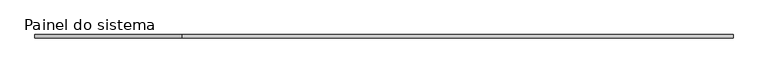
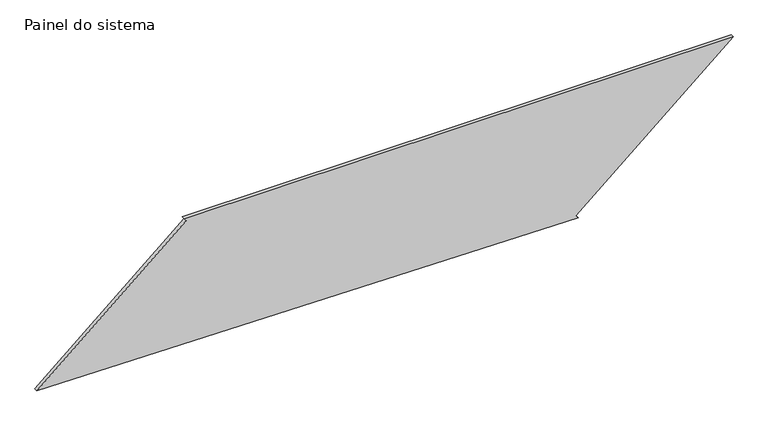
"""IFC4 building model written with IfcOpenShell, lengths in millimetres: plate geometry, Painel do sistema : Envidraçado."""

import ifcopenshell
import ifcopenshell.guid

model = None  # the IFC model being written
_history = None  # IfcOwnerHistory: only IFC2X3 demands one
_inside = {}  # id of a spatial element -> (the spatial element, [elements in it])
_under = {}  # id of a project, library or spatial element -> (it, [spatial elements below it])
_declared = {}  # id of a project -> (the project, [libraries it declares])
_typed = {}  # id of a type object -> (the type object, [elements of that type])
_made_of = {}  # id of a material, layer set ... -> (it, [elements and type objects made of it])


def new_model(schema):
    """Start an empty IFC model of exactly this schema.

    Asked for "IFC4X3", IfcOpenShell would pick the latest addendum, in which some entities
    have other attributes; the version numbers below select the first issue.
    IFC2X3 requires an IfcOwnerHistory on every rooted entity: one is made here for all.
    """
    global model, _history
    if schema == "IFC4X3":
        model = ifcopenshell.file(schema_version=(4, 3, 0, 0))
    else:
        model = ifcopenshell.file(schema=schema)
    _inside.clear()
    _under.clear()
    _declared.clear()
    _typed.clear()
    _made_of.clear()
    _history = None
    if model.schema == "IFC2X3":
        org = make("IfcOrganization", Name="unknown")
        user = make(
            "IfcPersonAndOrganization",
            ThePerson=make("IfcPerson", FamilyName="unknown"),
            TheOrganization=org,
        )
        app = make(
            "IfcApplication",
            ApplicationDeveloper=org,
            Version="unknown",
            ApplicationFullName="unknown",
            ApplicationIdentifier="unknown",
        )
        _history = make(
            "IfcOwnerHistory",
            OwningUser=user,
            OwningApplication=app,
            ChangeAction="ADDED",
            CreationDate=0,
        )
    return model


def make(cls, **values):
    """One entity of the class cls with the attributes given. An attribute that is None is left unset."""
    return model.create_entity(
        cls, **{name: value for name, value in values.items() if value is not None}
    )


def rooted(cls, **values):
    """An entity with a GlobalId (a new one), such as an element, a storey or a relation."""
    return make(cls, GlobalId=ifcopenshell.guid.new(), OwnerHistory=_history, **values)


def si_unit(unit_type, name, prefix=None):
    """IfcSIUnit, for example si_unit("LENGTHUNIT", "METRE", prefix="MILLI")."""
    return make("IfcSIUnit", UnitType=unit_type, Prefix=prefix, Name=name)


def assignment(units):
    """IfcUnitAssignment: the units of a project."""
    return None if units is None else make("IfcUnitAssignment", Units=units)


def point(xyz):
    """IfcCartesianPoint."""
    return None if xyz is None else make("IfcCartesianPoint", Coordinates=xyz)


def direction(xyz):
    """IfcDirection."""
    return None if xyz is None else make("IfcDirection", DirectionRatios=xyz)


def frame(location, z_axis=None, x_axis=None):
    """IfcAxis2Placement3D, a coordinate frame: its origin and axes. An axis left out is left unset."""
    return make(
        "IfcAxis2Placement3D",
        Location=point(location),
        Axis=direction(z_axis),
        RefDirection=direction(x_axis),
    )


def origin():
    """The frame at (0, 0, 0) with its axes left unset."""
    return frame((0.0, 0.0, 0.0))


def place(relative_to, where):
    """IfcLocalPlacement: puts the frame where relative to a parent placement (None: the world)."""
    return make(
        "IfcLocalPlacement", PlacementRelTo=relative_to, RelativePlacement=where
    )


def context(
    kind, dimensions, precision=None, world=None, true_north=None, identifier=None
):
    """IfcGeometricRepresentationContext, for example the 3D "Model" context."""
    return make(
        "IfcGeometricRepresentationContext",
        ContextIdentifier=identifier,
        ContextType=kind,
        CoordinateSpaceDimension=dimensions,
        Precision=precision,
        WorldCoordinateSystem=world,
        TrueNorth=true_north,
    )


def project(units=None, contexts=None):
    """IfcProject with its units and contexts."""
    return rooted(
        "IfcProject",
        Name="project",
        RepresentationContexts=contexts,
        UnitsInContext=assignment(units),
    )


def spatial(cls, under=None, at=None, **own):
    """A site, building, storey or space (cls), placed at a placement, below another one or the project."""
    s = rooted(cls, ObjectPlacement=at, **own)
    if under is not None:
        _under.setdefault(under.id(), (under, []))[1].append(s)
    return s


def polyline(points):
    """IfcPolyline through the points."""
    return make("IfcPolyline", Points=[point(p) for p in points])


def outline(outer, holes=None, kind="AREA"):
    """IfcArbitraryClosedProfileDef: a profile drawn as a closed curve; with holes, ...WithVoids."""
    if holes is None:
        return make("IfcArbitraryClosedProfileDef", ProfileType=kind, OuterCurve=outer)
    return make(
        "IfcArbitraryProfileDefWithVoids",
        ProfileType=kind,
        OuterCurve=outer,
        InnerCurves=holes,
    )


def extrude(swept, where, along, depth):
    """IfcExtrudedAreaSolid: the profile swept, set in the frame where, extruded along a direction by depth."""
    return make(
        "IfcExtrudedAreaSolid",
        SweptArea=swept,
        Position=where,
        ExtrudedDirection=direction(along),
        Depth=depth,
    )


def shape(context_of_items, identifier, shape_type, items):
    """IfcShapeRepresentation: the items that make up one representation, for example the "Body"."""
    return make(
        "IfcShapeRepresentation",
        ContextOfItems=context_of_items,
        RepresentationIdentifier=identifier,
        RepresentationType=shape_type,
        Items=items,
    )


def source(mapping_origin, context_of_items, identifier, shape_type, items):
    """IfcRepresentationMap: a shape defined once, which mapped items show again and again."""
    return make(
        "IfcRepresentationMap",
        MappingOrigin=mapping_origin,
        MappedRepresentation=shape(context_of_items, identifier, shape_type, items),
    )


def transform(
    local_origin,
    x_axis=None,
    y_axis=None,
    z_axis=None,
    scale=None,
    scale2=None,
    scale3=None,
    uniform=True,
):
    """IfcCartesianTransformationOperator3D, or its non-uniform kind. x_axis, y_axis, z_axis: its Axis1, 2, 3."""
    if uniform:
        return make(
            "IfcCartesianTransformationOperator3D",
            Axis1=direction(x_axis),
            Axis2=direction(y_axis),
            LocalOrigin=point(local_origin),
            Scale=scale,
            Axis3=direction(z_axis),
        )
    return make(
        "IfcCartesianTransformationOperator3DnonUniform",
        Axis1=direction(x_axis),
        Axis2=direction(y_axis),
        LocalOrigin=point(local_origin),
        Scale=scale,
        Axis3=direction(z_axis),
        Scale2=scale2,
        Scale3=scale3,
    )


def mapped(mapping_source, mapping_target):
    """IfcMappedItem: shows the shape of a source again, moved by a transform."""
    return make(
        "IfcMappedItem", MappingSource=mapping_source, MappingTarget=mapping_target
    )


def made_of(thing, what):
    """Note that an element or type object is made of a material, layer set ...; save() writes the relation."""
    if what is not None:
        _made_of.setdefault(what.id(), (what, []))[1].append(thing)
    return thing


def element(
    cls,
    number,
    at=None,
    inside=None,
    cuts=None,
    type_object=None,
    material=None,
    context=None,
    identifier="Body",
    shape_type=None,
    held_by="IfcProductDefinitionShape",
    body=None,
    shapes=None,
    **own,
):
    """One element of the class cls, such as IfcWall. Its Tag is "e" and its number.

    at: its placement. inside: the storey or other place that contains it. cuts: it is an
    opening in that element (IfcRelVoidsElement). A single representation is given by context,
    identifier, shape_type and body (its items); several are given by shapes. held_by: the class
    of the entity that holds the representations. save() writes the other relations.
    """
    e = rooted(cls, Tag="e%d" % number, ObjectPlacement=at, **own)
    if body is not None:
        shapes = [shape(context, identifier, shape_type, body)]
    if shapes is not None:
        e.Representation = make(held_by, Representations=shapes)
    if inside is not None:
        _inside.setdefault(inside.id(), (inside, []))[1].append(e)
    if cuts is not None:
        rooted(
            "IfcRelVoidsElement", RelatingBuildingElement=cuts, RelatedOpeningElement=e
        )
    if type_object is not None:
        _typed.setdefault(type_object.id(), (type_object, []))[1].append(e)
    return made_of(e, material)


def aggregate(whole, parts):
    """IfcRelAggregates: a whole, such as a stair, and the parts it consists of."""
    return rooted("IfcRelAggregates", RelatingObject=whole, RelatedObjects=parts)


def save(model, path):
    """Write the relations noted so far, then the file.

    IfcRelAggregates (storeys below a building ...), IfcRelContainedInSpatialStructure (elements
    in a storey), IfcRelDefinesByType, IfcRelAssociatesMaterial and IfcRelDeclares: one each for
    every whole, place, type object, material and project.
    """
    for whole, parts in _under.values():
        aggregate(whole, parts)
    for where, things in _inside.values():
        rooted(
            "IfcRelContainedInSpatialStructure",
            RelatedElements=things,
            RelatingStructure=where,
        )
    for kind, things in _typed.values():
        rooted("IfcRelDefinesByType", RelatedObjects=things, RelatingType=kind)
    for what, things in _made_of.values():
        rooted("IfcRelAssociatesMaterial", RelatedObjects=things, RelatingMaterial=what)
    for by, libraries in _declared.values():
        rooted("IfcRelDeclares", RelatingContext=by, RelatedDefinitions=libraries)
    model.write(path)


def painel_do_sistema_0a7026de(model_context):
    return source(origin(), model_context, "Body", "SweptSolid", [
        extrude(outline(polyline([(0.0, 1379.9338611), (19.0100862, 1363.6975862), (978.265335, 2486.8323592), (978.265335, -1435.9100035), (959.2552489, -1419.6737286), (47.8085175, -2486.8323592), (0.0, 1379.9338611)])), frame((0.0, 24.5, 0.0), z_axis=(0.0, 1.0, 0.0), x_axis=(0.0, 0.0, 1.0)), (0.0, 0.0, 1.0), 25.0),
    ])


if __name__ == "__main__":
    model = new_model("IFC4")
    model_context = context("Model", 3, world=origin())
    ifc_project = project(units=[si_unit("LENGTHUNIT", "METRE", prefix="MILLI")], contexts=[model_context])
    site = spatial("IfcSite", under=ifc_project)
    building = spatial("IfcBuilding", under=site)
    placement = place(None, origin())
    painel_do_sistema_shape = painel_do_sistema_0a7026de(model_context)
    element("IfcPlate", 1, ObjectType="Painel do sistema : Envidraçado", at=placement, inside=building, context=model_context, shape_type="MappedRepresentation", body=[
        mapped(painel_do_sistema_shape, transform((0.0, 0.0, 0.0), x_axis=(1.0, 0.0, 0.0), y_axis=(0.0, 1.0, 0.0), z_axis=(0.0, 0.0, 1.0))),
    ])
    save(model, "model.ifc")

# Revit data of these elements
# Type "Painel do sistema : Envidraçado"
#   Construction Type Id = "GSP4R"
#   Analytic Construction = "Vidraça única Pilkington 1/8 pol"
#   Visual Light Transmittance = 0.9
#   Solar Heat Gain Coefficient = 0.86
#   Heat Transfer Coefficient (U) = 6.7069 W/(m²·K)
# Element 1 (IfcPlate, "Painel do sistema : Envidraçado")
#   Materials on its faces: "Vidro"
# Materials
#   "Vidro": class "Vidro", colour RGB 0 128 192, transparency 0.9, Description = "Vidro de sílica", Cost = 0
